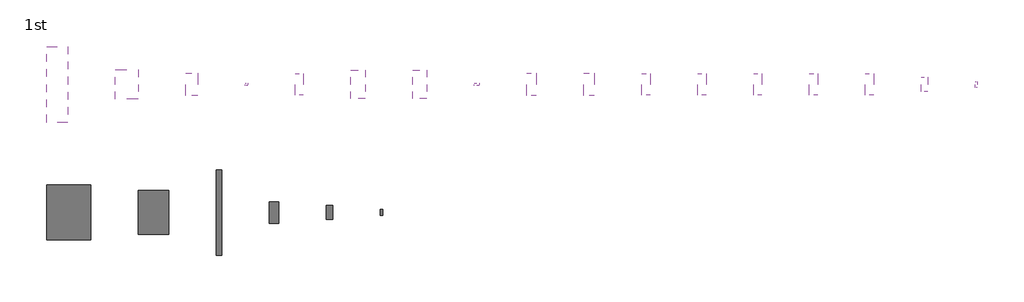
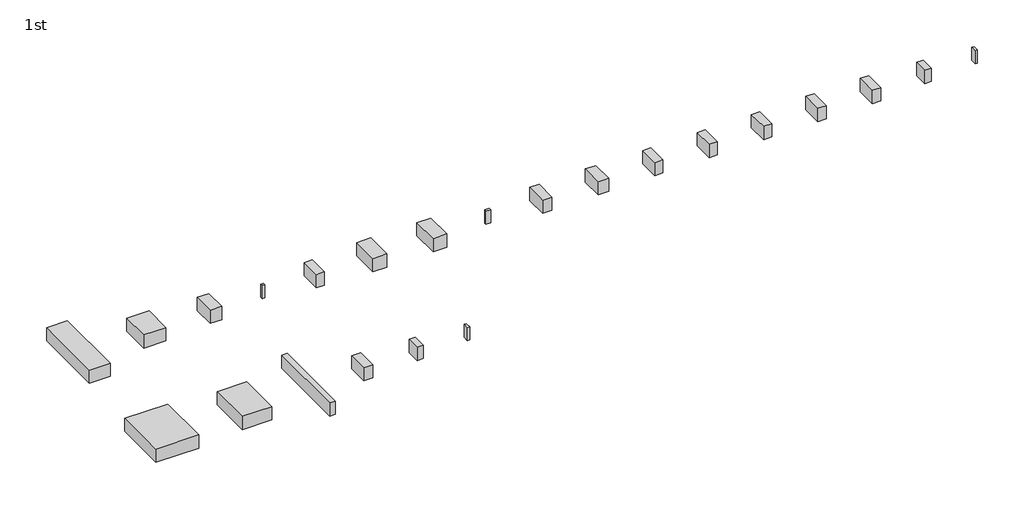
# One storey: 23 proxies.
"""IFC4 building model written with IfcOpenShell, lengths in millimetres."""

import ifcopenshell
import ifcopenshell.guid

model = None  # the IFC model being written
_history = None  # IfcOwnerHistory: only IFC2X3 demands one
_inside = {}  # id of a spatial element -> (the spatial element, [elements in it])
_under = {}  # id of a project, library or spatial element -> (it, [spatial elements below it])
_declared = {}  # id of a project -> (the project, [libraries it declares])
_typed = {}  # id of a type object -> (the type object, [elements of that type])
_made_of = {}  # id of a material, layer set ... -> (it, [elements and type objects made of it])


def new_model(schema):
    """Start an empty IFC model of exactly this schema.

    Asked for "IFC4X3", IfcOpenShell would pick the latest addendum, in which some entities
    have other attributes; the version numbers below select the first issue.
    IFC2X3 requires an IfcOwnerHistory on every rooted entity: one is made here for all.
    """
    global model, _history
    if schema == "IFC4X3":
        model = ifcopenshell.file(schema_version=(4, 3, 0, 0))
    else:
        model = ifcopenshell.file(schema=schema)
    _inside.clear()
    _under.clear()
    _declared.clear()
    _typed.clear()
    _made_of.clear()
    _history = None
    if model.schema == "IFC2X3":
        org = make("IfcOrganization", Name="unknown")
        user = make(
            "IfcPersonAndOrganization",
            ThePerson=make("IfcPerson", FamilyName="unknown"),
            TheOrganization=org,
        )
        app = make(
            "IfcApplication",
            ApplicationDeveloper=org,
            Version="unknown",
            ApplicationFullName="unknown",
            ApplicationIdentifier="unknown",
        )
        _history = make(
            "IfcOwnerHistory",
            OwningUser=user,
            OwningApplication=app,
            ChangeAction="ADDED",
            CreationDate=0,
        )
    return model


def make(cls, **values):
    """One entity of the class cls with the attributes given. An attribute that is None is left unset."""
    return model.create_entity(
        cls, **{name: value for name, value in values.items() if value is not None}
    )


def rooted(cls, **values):
    """An entity with a GlobalId (a new one), such as an element, a storey or a relation."""
    return make(cls, GlobalId=ifcopenshell.guid.new(), OwnerHistory=_history, **values)


def si_unit(unit_type, name, prefix=None):
    """IfcSIUnit, for example si_unit("LENGTHUNIT", "METRE", prefix="MILLI")."""
    return make("IfcSIUnit", UnitType=unit_type, Prefix=prefix, Name=name)


def assignment(units):
    """IfcUnitAssignment: the units of a project."""
    return None if units is None else make("IfcUnitAssignment", Units=units)


def point(xyz):
    """IfcCartesianPoint."""
    return None if xyz is None else make("IfcCartesianPoint", Coordinates=xyz)


def direction(xyz):
    """IfcDirection."""
    return None if xyz is None else make("IfcDirection", DirectionRatios=xyz)


def frame(location, z_axis=None, x_axis=None):
    """IfcAxis2Placement3D, a coordinate frame: its origin and axes. An axis left out is left unset."""
    return make(
        "IfcAxis2Placement3D",
        Location=point(location),
        Axis=direction(z_axis),
        RefDirection=direction(x_axis),
    )


def origin():
    """The frame at (0, 0, 0) with its axes left unset."""
    return frame((0.0, 0.0, 0.0))


def origin_with_axes():
    """The frame at (0, 0, 0) with the z axis (0, 0, 1) and the x axis (1, 0, 0) written out."""
    return frame((0.0, 0.0, 0.0), z_axis=(0.0, 0.0, 1.0), x_axis=(1.0, 0.0, 0.0))


def place(relative_to, where):
    """IfcLocalPlacement: puts the frame where relative to a parent placement (None: the world)."""
    return make(
        "IfcLocalPlacement", PlacementRelTo=relative_to, RelativePlacement=where
    )


def context(
    kind, dimensions, precision=None, world=None, true_north=None, identifier=None
):
    """IfcGeometricRepresentationContext, for example the 3D "Model" context."""
    return make(
        "IfcGeometricRepresentationContext",
        ContextIdentifier=identifier,
        ContextType=kind,
        CoordinateSpaceDimension=dimensions,
        Precision=precision,
        WorldCoordinateSystem=world,
        TrueNorth=true_north,
    )


def project(units=None, contexts=None):
    """IfcProject with its units and contexts."""
    return rooted(
        "IfcProject",
        Name="project",
        RepresentationContexts=contexts,
        UnitsInContext=assignment(units),
    )


def spatial(cls, under=None, at=None, **own):
    """A site, building, storey or space (cls), placed at a placement, below another one or the project."""
    s = rooted(cls, ObjectPlacement=at, **own)
    if under is not None:
        _under.setdefault(under.id(), (under, []))[1].append(s)
    return s


def polyline(points):
    """IfcPolyline through the points."""
    return make("IfcPolyline", Points=[point(p) for p in points])


def outline(outer, holes=None, kind="AREA"):
    """IfcArbitraryClosedProfileDef: a profile drawn as a closed curve; with holes, ...WithVoids."""
    if holes is None:
        return make("IfcArbitraryClosedProfileDef", ProfileType=kind, OuterCurve=outer)
    return make(
        "IfcArbitraryProfileDefWithVoids",
        ProfileType=kind,
        OuterCurve=outer,
        InnerCurves=holes,
    )


def extrude(swept, where, along, depth):
    """IfcExtrudedAreaSolid: the profile swept, set in the frame where, extruded along a direction by depth."""
    return make(
        "IfcExtrudedAreaSolid",
        SweptArea=swept,
        Position=where,
        ExtrudedDirection=direction(along),
        Depth=depth,
    )


def shape(context_of_items, identifier, shape_type, items):
    """IfcShapeRepresentation: the items that make up one representation, for example the "Body"."""
    return make(
        "IfcShapeRepresentation",
        ContextOfItems=context_of_items,
        RepresentationIdentifier=identifier,
        RepresentationType=shape_type,
        Items=items,
    )


def source(mapping_origin, context_of_items, identifier, shape_type, items):
    """IfcRepresentationMap: a shape defined once, which mapped items show again and again."""
    return make(
        "IfcRepresentationMap",
        MappingOrigin=mapping_origin,
        MappedRepresentation=shape(context_of_items, identifier, shape_type, items),
    )


def transform(
    local_origin,
    x_axis=None,
    y_axis=None,
    z_axis=None,
    scale=None,
    scale2=None,
    scale3=None,
    uniform=True,
):
    """IfcCartesianTransformationOperator3D, or its non-uniform kind. x_axis, y_axis, z_axis: its Axis1, 2, 3."""
    if uniform:
        return make(
            "IfcCartesianTransformationOperator3D",
            Axis1=direction(x_axis),
            Axis2=direction(y_axis),
            LocalOrigin=point(local_origin),
            Scale=scale,
            Axis3=direction(z_axis),
        )
    return make(
        "IfcCartesianTransformationOperator3DnonUniform",
        Axis1=direction(x_axis),
        Axis2=direction(y_axis),
        LocalOrigin=point(local_origin),
        Scale=scale,
        Axis3=direction(z_axis),
        Scale2=scale2,
        Scale3=scale3,
    )


def mapped(mapping_source, mapping_target):
    """IfcMappedItem: shows the shape of a source again, moved by a transform."""
    return make(
        "IfcMappedItem", MappingSource=mapping_source, MappingTarget=mapping_target
    )


def made_of(thing, what):
    """Note that an element or type object is made of a material, layer set ...; save() writes the relation."""
    if what is not None:
        _made_of.setdefault(what.id(), (what, []))[1].append(thing)
    return thing


def element(
    cls,
    number,
    at=None,
    inside=None,
    cuts=None,
    type_object=None,
    material=None,
    context=None,
    identifier="Body",
    shape_type=None,
    held_by="IfcProductDefinitionShape",
    body=None,
    shapes=None,
    **own,
):
    """One element of the class cls, such as IfcWall. Its Tag is "e" and its number.

    at: its placement. inside: the storey or other place that contains it. cuts: it is an
    opening in that element (IfcRelVoidsElement). A single representation is given by context,
    identifier, shape_type and body (its items); several are given by shapes. held_by: the class
    of the entity that holds the representations. save() writes the other relations.
    """
    e = rooted(cls, Tag="e%d" % number, ObjectPlacement=at, **own)
    if body is not None:
        shapes = [shape(context, identifier, shape_type, body)]
    if shapes is not None:
        e.Representation = make(held_by, Representations=shapes)
    if inside is not None:
        _inside.setdefault(inside.id(), (inside, []))[1].append(e)
    if cuts is not None:
        rooted(
            "IfcRelVoidsElement", RelatingBuildingElement=cuts, RelatedOpeningElement=e
        )
    if type_object is not None:
        _typed.setdefault(type_object.id(), (type_object, []))[1].append(e)
    return made_of(e, material)


def aggregate(whole, parts):
    """IfcRelAggregates: a whole, such as a stair, and the parts it consists of."""
    return rooted("IfcRelAggregates", RelatingObject=whole, RelatedObjects=parts)


def save(model, path):
    """Write the relations noted so far, then the file.

    IfcRelAggregates (storeys below a building ...), IfcRelContainedInSpatialStructure (elements
    in a storey), IfcRelDefinesByType, IfcRelAssociatesMaterial and IfcRelDeclares: one each for
    every whole, place, type object, material and project.
    """
    for whole, parts in _under.values():
        aggregate(whole, parts)
    for where, things in _inside.values():
        rooted(
            "IfcRelContainedInSpatialStructure",
            RelatedElements=things,
            RelatingStructure=where,
        )
    for kind, things in _typed.values():
        rooted("IfcRelDefinesByType", RelatedObjects=things, RelatingType=kind)
    for what, things in _made_of.values():
        rooted("IfcRelAssociatesMaterial", RelatedObjects=things, RelatingMaterial=what)
    for by, libraries in _declared.values():
        rooted("IfcRelDeclares", RelatingContext=by, RelatedDefinitions=libraries)
    model.write(path)


def generic_models_29bcd6f9(model_context):
    return source(origin(), model_context, "Body", "SweptSolid", [
        extrude(outline(polyline([(2000.0, 4500.0), (2000.0, -4500.0), (-2000.0, -4500.0), (-2000.0, 4500.0), (2000.0, 4500.0)])), origin_with_axes(), (0.0, 0.0, 1.0), 6000.0),
    ])


def generic_models_d82b1902(model_context):
    return source(origin(), model_context, "Body", "SweptSolid", [
        extrude(outline(polyline([(9300.0, 11600.0), (9300.0, -11600.0), (-9300.0, -11600.0), (-9300.0, 11600.0), (9300.0, 11600.0)])), origin_with_axes(), (0.0, 0.0, 1.0), 6000.0),
    ])


def generic_models_21711933(model_context):
    return source(origin(), model_context, "Body", "SweptSolid", [
        extrude(outline(polyline([(6400.0, 9300.0), (6400.0, -9300.0), (-6400.0, -9300.0), (-6400.0, 9300.0), (6400.0, 9300.0)])), origin_with_axes(), (0.0, 0.0, 1.0), 6000.0),
    ])


def generic_models_03d31222(model_context):
    return source(origin(), model_context, "Body", "SweptSolid", [
        extrude(outline(polyline([(1200.0, 18000.0), (1200.0, -18000.0), (-1200.0, -18000.0), (-1200.0, 18000.0), (1200.0, 18000.0)])), origin_with_axes(), (0.0, 0.0, 1.0), 6000.0),
    ])


def generic_models_5634f436(model_context):
    return source(origin(), model_context, "Body", "SweptSolid", [
        extrude(outline(polyline([(1350.0, 3000.0), (1350.0, -3000.0), (-1350.0, -3000.0), (-1350.0, 3000.0), (1350.0, 3000.0)])), origin_with_axes(), (0.0, 0.0, 1.0), 6000.0),
    ])


def generic_models_71e2440f(model_context):
    return source(origin(), model_context, "Body", "SweptSolid", [
        extrude(outline(polyline([(500.0, 1250.0), (500.0, -1250.0), (-500.0, -1250.0), (-500.0, 1250.0), (500.0, 1250.0)])), origin_with_axes(), (0.0, 0.0, 1.0), 6000.0),
    ])


def generic_models_57c7875f(model_context):
    return source(origin(), model_context, "Body", "SweptSolid", [
        extrude(outline(polyline([(4500.0, 16000.0), (4500.0, -16000.0), (-4500.0, -16000.0), (-4500.0, 16000.0), (4500.0, 16000.0)])), origin_with_axes(), (0.0, 0.0, 1.0), 6000.0),
    ])


def generic_models_72d488a7(model_context):
    return source(origin(), model_context, "Body", "SweptSolid", [
        extrude(outline(polyline([(4800.0, 6250.0), (4800.0, -6250.0), (-4800.0, -6250.0), (-4800.0, 6250.0), (4800.0, 6250.0)])), origin_with_axes(), (0.0, 0.0, 1.0), 6000.0),
    ])


def generic_models_7902148a(model_context):
    return source(origin(), model_context, "Body", "SweptSolid", [
        extrude(outline(polyline([(2500.0, 4800.0), (2500.0, -4800.0), (-2500.0, -4800.0), (-2500.0, 4800.0), (2500.0, 4800.0)])), origin_with_axes(), (0.0, 0.0, 1.0), 6000.0),
    ])


def generic_models_ed4b717c(model_context):
    return source(origin(), model_context, "Body", "SweptSolid", [
        extrude(outline(polyline([(500.0, 500.0), (500.0, -500.0), (-500.0, -500.0), (-500.0, 500.0), (500.0, 500.0)])), origin_with_axes(), (0.0, 0.0, 1.0), 6000.0),
    ])


def generic_models_c01b8d6f(model_context):
    return source(origin(), model_context, "Body", "SweptSolid", [
        extrude(outline(polyline([(1750.0, 4500.0), (1750.0, -4500.0), (-1750.0, -4500.0), (-1750.0, 4500.0), (1750.0, 4500.0)])), origin_with_axes(), (0.0, 0.0, 1.0), 6000.0),
    ])


def generic_models_43059f4e(model_context):
    return source(origin(), model_context, "Body", "SweptSolid", [
        extrude(outline(polyline([(3000.0, 6000.0), (3000.0, -6000.0), (-3000.0, -6000.0), (-3000.0, 6000.0), (3000.0, 6000.0)])), origin_with_axes(), (0.0, 0.0, 1.0), 6000.0),
    ])


def generic_models_da00a96f(model_context):
    return source(origin(), model_context, "Body", "SweptSolid", [
        extrude(outline(polyline([(1000.0, 500.0), (1000.0, -500.0), (-1000.0, -500.0), (-1000.0, 500.0), (1000.0, 500.0)])), origin_with_axes(), (0.0, 0.0, 1.0), 6000.0),
    ])


def generic_models_3a820573(model_context):
    return source(origin(), model_context, "Body", "SweptSolid", [
        extrude(outline(polyline([(2000.0, 4750.0), (2000.0, -4750.0), (-2000.0, -4750.0), (-2000.0, 4750.0), (2000.0, 4750.0)])), origin_with_axes(), (0.0, 0.0, 1.0), 6000.0),
    ])


def generic_models_96097b63(model_context):
    return source(origin(), model_context, "Body", "SweptSolid", [
        extrude(outline(polyline([(2250.0, 4800.0), (2250.0, -4800.0), (-2250.0, -4800.0), (-2250.0, 4800.0), (2250.0, 4800.0)])), origin_with_axes(), (0.0, 0.0, 1.0), 6000.0),
    ])


model = new_model("IFC4")

# Units and contexts
model_context = context("Model", 3, world=origin())
ifc_project = project(units=[si_unit("LENGTHUNIT", "METRE", prefix="MILLI")], contexts=[model_context])

# Site, building, storey
site = spatial("IfcSite", under=ifc_project)
building = spatial("IfcBuilding", under=site)
storey = spatial("IfcBuildingStorey", under=building, Name="1st", Elevation=6000.0)

# Proxies
placement = place(None, origin())
generic_models_shape = generic_models_29bcd6f9(model_context)
element("IfcBuildingElementProxy", 1, Name="Space Planning Box_hec : Space Planning Box_hec", ObjectType="Space Planning Box_hec : Space Planning Box_hec", at=placement, inside=storey, context=model_context, shape_type="MappedRepresentation", body=[
    mapped(generic_models_shape, transform((95800.0, 114000.0, 6000.0), x_axis=(1.0, 0.0, 0.0), y_axis=(0.0, 1.0, 0.0), z_axis=(0.0, 0.0, 1.0))),
])
generic_models_2_shape = generic_models_d82b1902(model_context)
element("IfcBuildingElementProxy", 2, Name="Space Planning Box_hec : Space Planning Box_hec", ObjectType="Space Planning Box_hec : Space Planning Box_hec", at=placement, inside=storey, context=model_context, shape_type="MappedRepresentation", body=[
    mapped(generic_models_2_shape, transform((9300.0, 114000.0, 6000.0), x_axis=(1.0, 0.0, 0.0), y_axis=(0.0, 1.0, 0.0), z_axis=(0.0, 0.0, 1.0))),
])
generic_models_3_shape = generic_models_21711933(model_context)
element("IfcBuildingElementProxy", 3, Name="Space Planning Box_hec : Space Planning Box_hec", ObjectType="Space Planning Box_hec : Space Planning Box_hec", at=placement, inside=storey, context=model_context, shape_type="MappedRepresentation", body=[
    mapped(generic_models_3_shape, transform((45000.0, 114000.0, 6000.0), x_axis=(1.0, 0.0, 0.0), y_axis=(0.0, 1.0, 0.0), z_axis=(0.0, 0.0, 1.0))),
])
generic_models_4_shape = generic_models_03d31222(model_context)
element("IfcBuildingElementProxy", 4, Name="Space Planning Box_hec : Space Planning Box_hec", ObjectType="Space Planning Box_hec : Space Planning Box_hec", at=placement, inside=storey, context=model_context, shape_type="MappedRepresentation", body=[
    mapped(generic_models_4_shape, transform((72600.0, 114000.0, 6000.0), x_axis=(1.0, 0.0, 0.0), y_axis=(0.0, 1.0, 0.0), z_axis=(0.0, 0.0, 1.0))),
])
generic_models_5_shape = generic_models_5634f436(model_context)
element("IfcBuildingElementProxy", 5, Name="Space Planning Box_hec : Space Planning Box_hec", ObjectType="Space Planning Box_hec : Space Planning Box_hec", at=placement, inside=storey, context=model_context, shape_type="MappedRepresentation", body=[
    mapped(generic_models_5_shape, transform((119150.0, 114000.0, 6000.0), x_axis=(1.0, 0.0, 0.0), y_axis=(0.0, 1.0, 0.0), z_axis=(0.0, 0.0, 1.0))),
])
element("IfcBuildingElementProxy", 6, Name="Space Planning Box_hec : Space Planning Box_hec", ObjectType="Space Planning Box_hec : Space Planning Box_hec", at=placement, inside=storey, context=model_context, shape_type="MappedRepresentation", body=[
    mapped(generic_models_5_shape, transform((369450.0, 168000.0, 12000.0), x_axis=(1.0, 0.0, 0.0), y_axis=(0.0, 1.0, 0.0), z_axis=(0.0, 0.0, 1.0))),
])
generic_models_6_shape = generic_models_71e2440f(model_context)
element("IfcBuildingElementProxy", 7, Name="Space Planning Box_hec : Space Planning Box_hec", ObjectType="Space Planning Box_hec : Space Planning Box_hec", at=placement, inside=storey, context=model_context, shape_type="MappedRepresentation", body=[
    mapped(generic_models_6_shape, transform((141000.0, 114000.0, 6000.0), x_axis=(1.0, 0.0, 0.0), y_axis=(0.0, 1.0, 0.0), z_axis=(0.0, 0.0, 1.0))),
])
element("IfcBuildingElementProxy", 8, Name="Space Planning Box_hec : Space Planning Box_hec", ObjectType="Space Planning Box_hec : Space Planning Box_hec", at=placement, inside=storey, context=model_context, shape_type="MappedRepresentation", body=[
    mapped(generic_models_6_shape, transform((391300.0, 168000.0, 12000.0), x_axis=(1.0, 0.0, 0.0), y_axis=(0.0, 1.0, 0.0), z_axis=(0.0, 0.0, 1.0))),
])
generic_models_7_shape = generic_models_57c7875f(model_context)
element("IfcBuildingElementProxy", 9, Name="Space Planning Box_hec : Space Planning Box_hec", ObjectType="Space Planning Box_hec : Space Planning Box_hec", at=placement, inside=storey, context=model_context, shape_type="MappedRepresentation", body=[
    mapped(generic_models_7_shape, transform((4500.0, 168000.0, 12000.0), x_axis=(1.0, 0.0, 0.0), y_axis=(0.0, 1.0, 0.0), z_axis=(0.0, 0.0, 1.0))),
])
generic_models_8_shape = generic_models_72d488a7(model_context)
element("IfcBuildingElementProxy", 10, Name="Space Planning Box_hec : Space Planning Box_hec", ObjectType="Space Planning Box_hec : Space Planning Box_hec", at=placement, inside=storey, context=model_context, shape_type="MappedRepresentation", body=[
    mapped(generic_models_8_shape, transform((33800.0, 168000.0, 12000.0), x_axis=(1.0, 0.0, 0.0), y_axis=(0.0, 1.0, 0.0), z_axis=(0.0, 0.0, 1.0))),
])
generic_models_9_shape = generic_models_7902148a(model_context)
element("IfcBuildingElementProxy", 11, Name="Space Planning Box_hec : Space Planning Box_hec", ObjectType="Space Planning Box_hec : Space Planning Box_hec", at=placement, inside=storey, context=model_context, shape_type="MappedRepresentation", body=[
    mapped(generic_models_9_shape, transform((61100.0, 168000.0, 12000.0), x_axis=(1.0, 0.0, 0.0), y_axis=(0.0, 1.0, 0.0), z_axis=(0.0, 0.0, 1.0))),
])
generic_models_10_shape = generic_models_ed4b717c(model_context)
element("IfcBuildingElementProxy", 12, Name="Space Planning Box_hec : Space Planning Box_hec", ObjectType="Space Planning Box_hec : Space Planning Box_hec", at=placement, inside=storey, context=model_context, shape_type="MappedRepresentation", body=[
    mapped(generic_models_10_shape, transform((84100.0, 168000.0, 12000.0), x_axis=(1.0, 0.0, 0.0), y_axis=(0.0, 1.0, 0.0), z_axis=(0.0, 0.0, 1.0))),
])
generic_models_11_shape = generic_models_c01b8d6f(model_context)
element("IfcBuildingElementProxy", 13, Name="Space Planning Box_hec : Space Planning Box_hec", ObjectType="Space Planning Box_hec : Space Planning Box_hec", at=placement, inside=storey, context=model_context, shape_type="MappedRepresentation", body=[
    mapped(generic_models_11_shape, transform((106350.0, 168000.0, 12000.0), x_axis=(1.0, 0.0, 0.0), y_axis=(0.0, 1.0, 0.0), z_axis=(0.0, 0.0, 1.0))),
])
element("IfcBuildingElementProxy", 14, Name="Space Planning Box_hec : Space Planning Box_hec", ObjectType="Space Planning Box_hec : Space Planning Box_hec", at=placement, inside=storey, context=model_context, shape_type="MappedRepresentation", body=[
    mapped(generic_models_11_shape, transform((252350.0, 168000.0, 12000.0), x_axis=(1.0, 0.0, 0.0), y_axis=(0.0, 1.0, 0.0), z_axis=(0.0, 0.0, 1.0))),
])
element("IfcBuildingElementProxy", 15, Name="Space Planning Box_hec : Space Planning Box_hec", ObjectType="Space Planning Box_hec : Space Planning Box_hec", at=placement, inside=storey, context=model_context, shape_type="MappedRepresentation", body=[
    mapped(generic_models_11_shape, transform((275850.0, 168000.0, 12000.0), x_axis=(1.0, 0.0, 0.0), y_axis=(0.0, 1.0, 0.0), z_axis=(0.0, 0.0, 1.0))),
])
element("IfcBuildingElementProxy", 16, Name="Space Planning Box_hec : Space Planning Box_hec", ObjectType="Space Planning Box_hec : Space Planning Box_hec", at=placement, inside=storey, context=model_context, shape_type="MappedRepresentation", body=[
    mapped(generic_models_11_shape, transform((299350.0, 168000.0, 12000.0), x_axis=(1.0, 0.0, 0.0), y_axis=(0.0, 1.0, 0.0), z_axis=(0.0, 0.0, 1.0))),
])
element("IfcBuildingElementProxy", 17, Name="Space Planning Box_hec : Space Planning Box_hec", ObjectType="Space Planning Box_hec : Space Planning Box_hec", at=placement, inside=storey, context=model_context, shape_type="MappedRepresentation", body=[
    mapped(generic_models_11_shape, transform((322850.0, 168000.0, 12000.0), x_axis=(1.0, 0.0, 0.0), y_axis=(0.0, 1.0, 0.0), z_axis=(0.0, 0.0, 1.0))),
])
element("IfcBuildingElementProxy", 18, Name="Space Planning Box_hec : Space Planning Box_hec", ObjectType="Space Planning Box_hec : Space Planning Box_hec", at=placement, inside=storey, context=model_context, shape_type="MappedRepresentation", body=[
    mapped(generic_models_11_shape, transform((346350.0, 168000.0, 12000.0), x_axis=(1.0, 0.0, 0.0), y_axis=(0.0, 1.0, 0.0), z_axis=(0.0, 0.0, 1.0))),
])
generic_models_12_shape = generic_models_43059f4e(model_context)
element("IfcBuildingElementProxy", 19, Name="Space Planning Box_hec : Space Planning Box_hec", ObjectType="Space Planning Box_hec : Space Planning Box_hec", at=placement, inside=storey, context=model_context, shape_type="MappedRepresentation", body=[
    mapped(generic_models_12_shape, transform((131100.0, 168000.0, 12000.0), x_axis=(1.0, 0.0, 0.0), y_axis=(0.0, 1.0, 0.0), z_axis=(0.0, 0.0, 1.0))),
])
element("IfcBuildingElementProxy", 20, Name="Space Planning Box_hec : Space Planning Box_hec", ObjectType="Space Planning Box_hec : Space Planning Box_hec", at=placement, inside=storey, context=model_context, shape_type="MappedRepresentation", body=[
    mapped(generic_models_12_shape, transform((157100.0, 168000.0, 12000.0), x_axis=(1.0, 0.0, 0.0), y_axis=(0.0, 1.0, 0.0), z_axis=(0.0, 0.0, 1.0))),
])
generic_models_13_shape = generic_models_da00a96f(model_context)
element("IfcBuildingElementProxy", 21, Name="Space Planning Box_hec : Space Planning Box_hec", ObjectType="Space Planning Box_hec : Space Planning Box_hec", at=placement, inside=storey, context=model_context, shape_type="MappedRepresentation", body=[
    mapped(generic_models_13_shape, transform((181100.0, 168000.0, 12000.0), x_axis=(1.0, 0.0, 0.0), y_axis=(0.0, 1.0, 0.0), z_axis=(0.0, 0.0, 1.0))),
])
generic_models_14_shape = generic_models_3a820573(model_context)
element("IfcBuildingElementProxy", 22, Name="Space Planning Box_hec : Space Planning Box_hec", ObjectType="Space Planning Box_hec : Space Planning Box_hec", at=placement, inside=storey, context=model_context, shape_type="MappedRepresentation", body=[
    mapped(generic_models_14_shape, transform((204100.0, 168000.0, 12000.0), x_axis=(1.0, 0.0, 0.0), y_axis=(0.0, 1.0, 0.0), z_axis=(0.0, 0.0, 1.0))),
])
generic_models_15_shape = generic_models_96097b63(model_context)
element("IfcBuildingElementProxy", 23, Name="Space Planning Box_hec : Space Planning Box_hec", ObjectType="Space Planning Box_hec : Space Planning Box_hec", at=placement, inside=storey, context=model_context, shape_type="MappedRepresentation", body=[
    mapped(generic_models_15_shape, transform((228350.0, 168000.0, 12000.0), x_axis=(1.0, 0.0, 0.0), y_axis=(0.0, 1.0, 0.0), z_axis=(0.0, 0.0, 1.0))),
])

save(model, "model.ifc")

# Revit data of these elements
# Project information
#   Building Name = "MAIN GATE SECURITY BUILDING"
#   Project Status = "Project Status"
#   Client Name = "현대엔지니어링"
#   Project Address = "서울시 종로구 율곡로 75(계동)"
#   Project Name = "Therma Visayas Energy Project"
#   Project Number = "-"
# Grids (mm)
#   "A": line (45459.652, 190234.526) -> (45459.652, 152139.384)
#   "B": line (53459.652, 190234.526) -> (53459.652, 152139.384)
#   "C": line (61459.652, 190234.526) -> (61459.652, 152139.384)
#   "D": line (67459.652, 190234.526) -> (67459.652, 152139.384)
#   "E": line (73459.652, 190234.526) -> (73459.652, 152139.384)
#   "F": line (81459.652, 190234.526) -> (81459.652, 152139.384)
#   "G": line (85459.652, 190234.526) -> (85459.652, 152139.384)
#   "H": line (89459.652, 190234.526) -> (89459.652, 152139.384)
#   "4": line (39389.066, 184923.861) -> (102402.798, 184923.861)
#   "3": line (39389.066, 178923.861) -> (102402.798, 178923.861)
#   "2": line (39389.066, 172923.861) -> (102402.798, 172923.861)
#   "1": line (39389.066, 163923.861) -> (102402.798, 163923.861)
# Type "Space Planning Box_hec : Space Planning Box_hec"
#   Type Comments = "..."
#   Room Name [instance default] = "?"
#   Interior Finish [instance default] = ""
#   Exterior Finish [instance default] = ""
#   Department [instance default] = ""
#   Assembly Code = "..."
#   Width [instance default] = 1524 mm
#   Program Area [instance default] = 0.00 m²
#   Length [instance default] = 1524 mm
#   Height [instance default] = 1524 mm
#   Area [instance default] = 2.32258 m²
#   Fill Color [instance default] = Cyan
#   Default Elevation = 0
# Element 1 (IfcBuildingElementProxy, "Space Planning Box_hec : Space Planning Box_hec")
#   Room Name = "Stairway"
#   Interior Finish = "IF2"
#   Exterior Finish = "EF1"
#   Department = "AR"
#   Width = 4000 mm
#   Program Area = 36.00 m²
#   Length = 9000 mm
#   Height = 6000 mm
#   Area = 36.00 m²
#   Fill Color = Lavender
#   Phase Created = New Construction
#   Materials on its faces: "Lavender"
# Element 2 (IfcBuildingElementProxy, "Space Planning Box_hec : Space Planning Box_hec")
#   Room Name = "Electronic Room"
#   Interior Finish = "IF1"
#   Exterior Finish = "EF1"
#   Department = "CI"
#   Width = 18600 mm
#   Program Area = 431.52 m²
#   Length = 23200 mm
#   Height = 6000 mm
#   Area = 431.52 m²
#   Fill Color = Lime
#   Phase Created = New Construction
#   Materials on its faces: "Lime"
# Element 3 (IfcBuildingElementProxy, "Space Planning Box_hec : Space Planning Box_hec")
#   Room Name = "Electrical Room"
#   Interior Finish = "IF1"
#   Exterior Finish = "EF1"
#   Department = "EL"
#   Width = 12800 mm
#   Program Area = 238.08 m²
#   Length = 18600 mm
#   Height = 6000 mm
#   Area = 238.08 m²
#   Fill Color = Blue
#   Phase Created = New Construction
#   Materials on its faces: "Blue"
# Element 4 (IfcBuildingElementProxy, "Space Planning Box_hec : Space Planning Box_hec")
#   Room Name = "Corridor"
#   Interior Finish = "IF2-1"
#   Exterior Finish = "EF1"
#   Department = "AR"
#   Width = 2400 mm
#   Program Area = 86.40 m²
#   Length = 36000 mm
#   Height = 6000 mm
#   Area = 86.40 m²
#   Fill Color = Lavender
#   Phase Created = New Construction
#   Materials on its faces: "Lavender"
# Elements 5, 6 (IfcBuildingElementProxy, "Space Planning Box_hec : Space Planning Box_hec")
#   Room Name = "Duct Shaft"
#   Interior Finish = "NA"
#   Exterior Finish = "EF1"
#   Department = "HV"
#   Width = 2700 mm
#   Program Area = 16.20 m²
#   Length = 6000 mm
#   Height = 6000 mm
#   Area = 16.20 m²
#   Fill Color = Pink
#   Phase Created = New Construction
#   Materials on its faces: "Pink"
# Elements 7, 8 (IfcBuildingElementProxy, "Space Planning Box_hec : Space Planning Box_hec")
#   Room Name = "Pipe Shaft"
#   Interior Finish = "NA"
#   Exterior Finish = "EF1"
#   Department = "HV"
#   Width = 1000 mm
#   Program Area = 2.50 m²
#   Length = 2500 mm
#   Height = 6000 mm
#   Area = 2.50 m²
#   Fill Color = Pink
#   Phase Created = New Construction
#   Materials on its faces: "Pink"
# Element 9 (IfcBuildingElementProxy, "Space Planning Box_hec : Space Planning Box_hec")
#   Room Name = "Central Control Room"
#   Interior Finish = "IF3"
#   Exterior Finish = "EF1"
#   Department = "CI"
#   Width = 9000 mm
#   Program Area = 288.00 m²
#   Length = 32000 mm
#   Height = 6000 mm
#   Area = 288.00 m²
#   Fill Color = Lime
#   Phase Created = New Construction
#   Materials on its faces: "Lime"
# Element 10 (IfcBuildingElementProxy, "Space Planning Box_hec : Space Planning Box_hec")
#   Room Name = "Engineer Room"
#   Interior Finish = "IF3"
#   Exterior Finish = "EF1"
#   Department = "CI"
#   Width = 9600 mm
#   Program Area = 120.00 m²
#   Length = 12500 mm
#   Height = 6000 mm
#   Area = 120.00 m²
#   Fill Color = Lime
#   Phase Created = New Construction
#   Materials on its faces: "Lime"
# Element 11 (IfcBuildingElementProxy, "Space Planning Box_hec : Space Planning Box_hec")
#   Room Name = "Document Room"
#   Interior Finish = "IF2-1"
#   Exterior Finish = "EF1"
#   Department = "AR"
#   Width = 5000 mm
#   Program Area = 48.00 m²
#   Length = 9600 mm
#   Height = 6000 mm
#   Area = 48.00 m²
#   Fill Color = Lavender
#   Phase Created = New Construction
#   Materials on its faces: "Lavender"
# Element 12 (IfcBuildingElementProxy, "Space Planning Box_hec : Space Planning Box_hec")
#   Room Name = "Fire Gas Room"
#   Interior Finish = "IF1"
#   Exterior Finish = "EF1"
#   Department = "SF"
#   Width = 1000 mm
#   Program Area = 0.00 m²
#   Length = 1000 mm
#   Height = 6000 mm
#   Area = 1.00 m²
#   Fill Color = Cyan
#   Phase Created = New Construction
#   Materials on its faces: "Cyan"
# Element 13 (IfcBuildingElementProxy, "Space Planning Box_hec : Space Planning Box_hec")
#   Room Name = "Kitch & Lunch Room"
#   Interior Finish = "IF2-1"
#   Exterior Finish = "EF1"
#   Department = "AR"
#   Width = 3500 mm
#   Program Area = 31.50 m²
#   Length = 9000 mm
#   Height = 6000 mm
#   Area = 31.50 m²
#   Fill Color = Lavender
#   Phase Created = New Construction
#   Materials on its faces: "Lavender"
# Element 14 (IfcBuildingElementProxy, "Space Planning Box_hec : Space Planning Box_hec")
#   Room Name = "LOTO Office Room"
#   Interior Finish = "IF2-1"
#   Exterior Finish = "EF1"
#   Department = "AR"
#   Width = 3500 mm
#   Program Area = 31.50 m²
#   Length = 9000 mm
#   Height = 6000 mm
#   Area = 31.50 m²
#   Fill Color = Lavender
#   Phase Created = New Construction
#   Materials on its faces: "Lavender"
# Element 15 (IfcBuildingElementProxy, "Space Planning Box_hec : Space Planning Box_hec")
#   Room Name = "Shower Room (F)"
#   Interior Finish = "IF5"
#   Exterior Finish = "EF1"
#   Department = "AR"
#   Width = 3500 mm
#   Program Area = 31.50 m²
#   Length = 9000 mm
#   Height = 6000 mm
#   Area = 31.50 m²
#   Fill Color = Lavender
#   Phase Created = New Construction
#   Materials on its faces: "Lavender"
# Element 16 (IfcBuildingElementProxy, "Space Planning Box_hec : Space Planning Box_hec")
#   Room Name = "Locker Room (F)"
#   Interior Finish = "IF2-1"
#   Exterior Finish = "EF1"
#   Department = "AR"
#   Width = 3500 mm
#   Program Area = 31.50 m²
#   Length = 9000 mm
#   Height = 6000 mm
#   Area = 31.50 m²
#   Fill Color = Lavender
#   Phase Created = New Construction
#   Materials on its faces: "Lavender"
# Element 17 (IfcBuildingElementProxy, "Space Planning Box_hec : Space Planning Box_hec")
#   Room Name = "Shower Room (M)"
#   Interior Finish = "IF5"
#   Exterior Finish = "EF1"
#   Department = "AR"
#   Width = 3500 mm
#   Program Area = 31.50 m²
#   Length = 9000 mm
#   Height = 6000 mm
#   Area = 31.50 m²
#   Fill Color = Lavender
#   Phase Created = New Construction
#   Materials on its faces: "Lavender"
# Element 18 (IfcBuildingElementProxy, "Space Planning Box_hec : Space Planning Box_hec")
#   Room Name = "Locker Room (M)"
#   Interior Finish = "IF2-1"
#   Exterior Finish = "EF1"
#   Department = "AR"
#   Width = 3500 mm
#   Program Area = 31.50 m²
#   Length = 9000 mm
#   Height = 6000 mm
#   Area = 31.50 m²
#   Fill Color = Lavender
#   Phase Created = New Construction
#   Materials on its faces: "Lavender"
# Element 19 (IfcBuildingElementProxy, "Space Planning Box_hec : Space Planning Box_hec")
#   Room Name = "Toilet (M)"
#   Interior Finish = "IF5"
#   Exterior Finish = "EF1"
#   Department = "AR"
#   Width = 6000 mm
#   Program Area = 72.00 m²
#   Length = 12000 mm
#   Height = 6000 mm
#   Area = 72.00 m²
#   Fill Color = Lavender
#   Phase Created = New Construction
#   Materials on its faces: "Lavender"
# Element 20 (IfcBuildingElementProxy, "Space Planning Box_hec : Space Planning Box_hec")
#   Room Name = "Toilet (F)"
#   Interior Finish = "IF5"
#   Exterior Finish = "EF1"
#   Department = "AR"
#   Width = 6000 mm
#   Program Area = 72.00 m²
#   Length = 12000 mm
#   Height = 6000 mm
#   Area = 72.00 m²
#   Fill Color = Lavender
#   Phase Created = New Construction
#   Materials on its faces: "Lavender"
# Element 21 (IfcBuildingElementProxy, "Space Planning Box_hec : Space Planning Box_hec")
#   Room Name = "Corridor"
#   Interior Finish = "IF2-1"
#   Exterior Finish = "EF1"
#   Department = "AR"
#   Width = 2000 mm
#   Program Area = 0.00 m²
#   Length = 1000 mm
#   Height = 6000 mm
#   Area = 2.00 m²
#   Fill Color = Lavender
#   Phase Created = New Construction
#   Materials on its faces: "Lavender"
# Element 22 (IfcBuildingElementProxy, "Space Planning Box_hec : Space Planning Box_hec")
#   Room Name = "Stairway"
#   Interior Finish = "IF2"
#   Exterior Finish = "EF1"
#   Department = "AR"
#   Width = 4000 mm
#   Program Area = 38.00 m²
#   Length = 9500 mm
#   Height = 6000 mm
#   Area = 38.00 m²
#   Fill Color = Lavender
#   Phase Created = New Construction
#   Materials on its faces: "Lavender"
# Element 23 (IfcBuildingElementProxy, "Space Planning Box_hec : Space Planning Box_hec")
#   Room Name = "Shift Office Room"
#   Interior Finish = "IF2-1"
#   Exterior Finish = "EF1"
#   Department = "AR"
#   Width = 4500 mm
#   Program Area = 43.20 m²
#   Length = 9600 mm
#   Height = 6000 mm
#   Area = 43.20 m²
#   Fill Color = Lavender
#   Phase Created = New Construction
#   Materials on its faces: "Lavender"
# Materials
#   "Cyan": class "Generic", colour RGB 0 255 255, transparency 0.2, Cost = 0
#   "Lavender": class "Generic", colour RGB 186 85 211, transparency 0.2, Cost = 0
#   "Lime": class "Generic", colour RGB 0 255 0, transparency 0.2, Cost = 0
#   "Blue": class "Generic", colour RGB 0 0 255, transparency 0.2, Cost = 0
#   "Pink": class "Generic", colour RGB 255 105 180, transparency 0.2, Cost = 0
